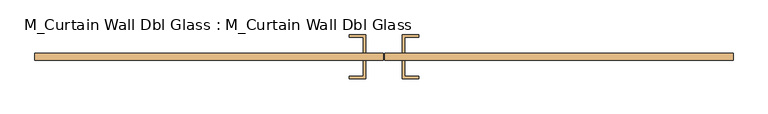
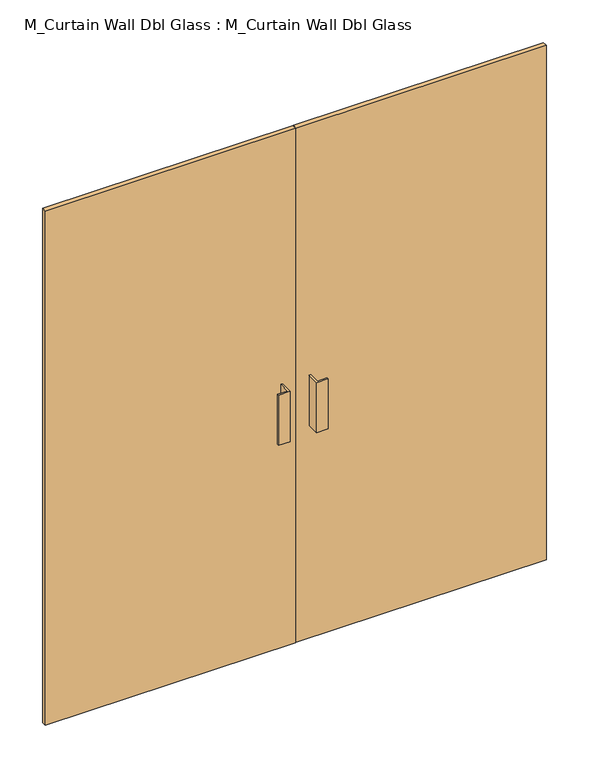
"""IFC4 building model written with IfcOpenShell, lengths in millimetres: door geometry, M_Curtain Wall Dbl Glass : M_Curtain Wall Dbl Glass."""

from ifc_helpers import new_model, si_unit, frame, origin, origin_with_axes, place, context, project, spatial, polyline, outline, extrude, source, transform, mapped, element, save


def m_curtain_wall_dbl_glass_m_curtain_wall_dbl_glass_a8ce7090(model_context):
    return source(origin(), model_context, "Body", "SweptSolid", [
        extrude(outline(polyline([(-1.5875, 30.95), (-960.9584499, 30.95), (-960.9584499, 50.0), (-1.5875, 50.0), (-1.5875, 30.95)])), origin_with_axes(), (0.0, 0.0, 1.0), 2085.0),
        extrude(outline(polyline([(960.9584499, 30.95), (1.5875, 30.95), (1.5875, 50.0), (960.9584499, 50.0), (960.9584499, 30.95)])), origin_with_axes(), (0.0, 0.0, 1.0), 2085.0),
        extrude(outline(polyline([(-50.8, 100.8), (-50.8, 50.0), (-57.15, 50.0), (-57.15, 94.45), (-95.25, 94.45), (-95.25, 100.8), (-50.8, 100.8)])), frame((0.0, 0.0, 863.6), z_axis=(0.0, 0.0, 1.0), x_axis=(1.0, 0.0, 0.0)), (0.0, 0.0, 1.0), 203.2),
        extrude(outline(polyline([(50.8, 100.8), (95.25, 100.8), (95.25, 94.45), (57.15, 94.45), (57.15, 50.0), (50.8, 50.0), (50.8, 100.8)])), frame((0.0, 0.0, 863.6), z_axis=(0.0, 0.0, 1.0), x_axis=(1.0, 0.0, 0.0)), (0.0, 0.0, 1.0), 203.2),
        extrude(outline(polyline([(-50.8, -19.85), (-95.25, -19.85), (-95.25, -13.5), (-57.15, -13.5), (-57.15, 30.95), (-50.8, 30.95), (-50.8, -19.85)])), frame((0.0, 0.0, 863.6), z_axis=(0.0, 0.0, 1.0), x_axis=(1.0, 0.0, 0.0)), (0.0, 0.0, 1.0), 203.2),
        extrude(outline(polyline([(50.8, -19.85), (50.8, 30.95), (57.15, 30.95), (57.15, -13.5), (95.25, -13.5), (95.25, -19.85), (50.8, -19.85)])), frame((0.0, 0.0, 863.6), z_axis=(0.0, 0.0, 1.0), x_axis=(1.0, 0.0, 0.0)), (0.0, 0.0, 1.0), 203.2),
    ])


if __name__ == "__main__":
    model = new_model("IFC4")
    model_context = context("Model", 3, world=origin())
    ifc_project = project(units=[si_unit("LENGTHUNIT", "METRE", prefix="MILLI")], contexts=[model_context])
    site = spatial("IfcSite", under=ifc_project)
    building = spatial("IfcBuilding", under=site)
    placement = place(None, origin())
    m_curtain_wall_dbl_glass_m_curtain_wall_dbl_glass_shape = m_curtain_wall_dbl_glass_m_curtain_wall_dbl_glass_a8ce7090(model_context)
    element("IfcDoor", 1, ObjectType="M_Curtain Wall Dbl Glass : M_Curtain Wall Dbl Glass", at=placement, inside=building, context=model_context, shape_type="MappedRepresentation", body=[
        mapped(m_curtain_wall_dbl_glass_m_curtain_wall_dbl_glass_shape, transform((0.0, 0.0, 0.0), x_axis=(1.0, 0.0, 0.0), y_axis=(0.0, 1.0, 0.0), z_axis=(0.0, 0.0, 1.0))),
    ])
    save(model, "model.ifc")

# Revit data of these elements
# Type "M_Curtain Wall Dbl Glass : M_Curtain Wall Dbl Glass"
#   Model = "12345678"
#   Manufacturer = "Dublin Doors"
#   Description = "Double Glass Door"
#   Type Mark = "41"
#   COBie.Type.CreatedBy = "design@eagle.com"
#   COBie.Type.CreatedOn = "2016-09-13T05:47:35"
#   COBie.Type.Name = "Doors_M_Curtain Wall Dbl Glass_M_Curtain Wall Dbl Glass"
#   COBie.Type.Category = "23-30 10 00 : Doors"
#   COBie.Type.Description = "Double Glass Door"
#   COBie.Type.Manufacturer = "Dublin Doors"
#   COBie.Type.ModelNumber = "12345678"
#   Construction Type Id = "GSP4R"
#   Analytic Construction = "1/8 in Pilkington single glazing"
#   COBie.Type.ReplacementCost = 0
#   Visual Light Transmittance = 0.9
#   Solar Heat Gain Coefficient = 0.78
#   Offset = 50 mm
#   Heat Transfer Coefficient (U) = 3.6886 W/(m²·K)
#   COBie.Type = yes
#   Function = 1
#   Glazing Material = Glass
# Element 1 (IfcDoor, "M_Curtain Wall Dbl Glass : M_Curtain Wall Dbl Glass")
#   Materials on its faces: "Aluminum", "Glass"
# Materials
#   "Glass": class "Glass", colour RGB 0 128 192, transparency 0.75, Description = "Soda Lime Glass", Cost = 0
#   "Aluminum": class "Metal", colour RGB 247 247 247, transparency 0, Description = "Aluminum 6061", Cost = 0
